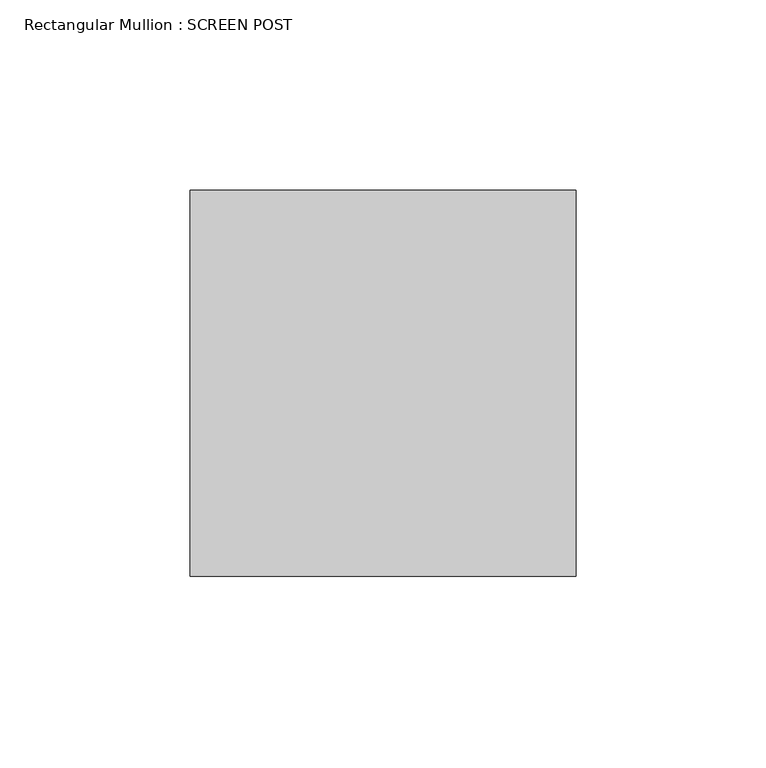
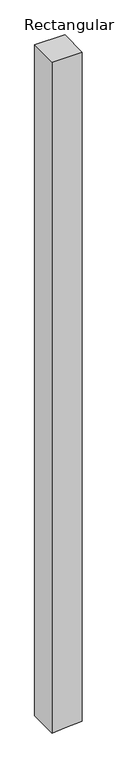
"""IFC4 building model written with IfcOpenShell, lengths in millimetres: member geometry, Rectangular Mullion : SCREEN POST."""

from ifc_helpers import new_model, si_unit, frame, origin, place, context, project, spatial, polyline, outline, extrude, source, transform, mapped, element, save


def rectangular_mullion_screen_post_9a11dd15(model_context):
    return source(origin(), model_context, "Body", "SweptSolid", [
        extrude(outline(polyline([(0.0, 50.8), (0.0, -50.8), (-2392.0540408, -50.8), (-2389.2708365, -6.3490391), (-2385.6925686, 50.8), (0.0, 50.8)])), frame((0.0, -50.8, 0.0), z_axis=(0.0, 1.0, 0.0), x_axis=(0.0, 0.0, 1.0)), (0.0, 0.0, 1.0), 101.6),
    ])


if __name__ == "__main__":
    model = new_model("IFC4")
    model_context = context("Model", 3, world=origin())
    ifc_project = project(units=[si_unit("LENGTHUNIT", "METRE", prefix="MILLI")], contexts=[model_context])
    site = spatial("IfcSite", under=ifc_project)
    building = spatial("IfcBuilding", under=site)
    placement = place(None, origin())
    rectangular_mullion_screen_post_shape = rectangular_mullion_screen_post_9a11dd15(model_context)
    element("IfcMember", 1, ObjectType="Rectangular Mullion : SCREEN POST", at=placement, inside=building, context=model_context, shape_type="MappedRepresentation", body=[
        mapped(rectangular_mullion_screen_post_shape, transform((0.0, 0.0, 0.0), x_axis=(1.0, 0.0, 0.0), y_axis=(0.0, 1.0, 0.0), z_axis=(0.0, 0.0, 1.0))),
    ])
    save(model, "model.ifc")

# Revit data of these elements
# Type "Rectangular Mullion : SCREEN POST"
#   built-in parameter 1007304 = 0.333333 (stored number, unit not read)
#   built-in parameter 1007301 = 0.166667 (stored number, unit not read)
#   built-in parameter 1007300 = 0.166667 (stored number, unit not read)
# Element 1 (IfcMember, "Rectangular Mullion : SCREEN POST")
#   Materials on its faces: "GLULAMS COLUMNS\n(PRESSURE TREATED W/ PENTA IN SOLVENT) (EXTERIOR STAIN: PENOFIN VERDE EXT. STAIN - COLOR: CEDAR)"
# Materials
#   "GLULAMS COLUMNS\n(PRESSURE TREATED W/ PENTA IN SOLVENT) (EXTERIOR STAIN: PENOFIN VERDE EXT. STAIN - COLOR: CEDAR)": class "Wood", colour RGB 164 134 123, transparency 0, Description = "Pinus Echinata", Cost = 0
